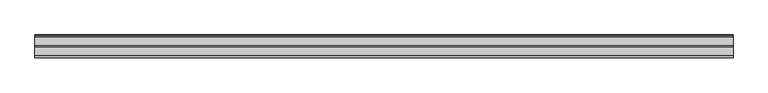
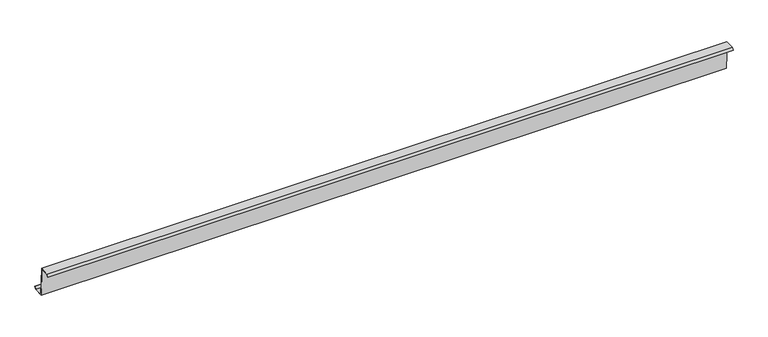
"""IFC4 building model written with IfcOpenShell, lengths in millimetres: proxy geometry, Generic Models 7:Generic Models 1:8:Generic Models 1:8 : Generic Models 7:Generic Models 1:337419:2 : Generic Models 7:Generic Models 1:8:Generic Models 1:8 : Generic Models 7:Generic Models 1:337419:315935."""

from ifc_helpers import new_model, si_unit, frame, origin, place, context, project, spatial, polyline, outline, extrude, source, transform, mapped, element, save


def generic_models_7addb1c7(model_context):
    return source(origin(), model_context, "Body", "SweptSolid", [
        extrude(outline(polyline([(-576223.748304, 4007.2948463), (-576158.9154956, 4009.9962133), (-576150.5718238, 3809.7480894), (-576089.8090698, 3812.2798708), (-576078.9727731, 3826.3439503), (-576076.7721093, 3824.6483508), (-576088.3990771, 3809.558085), (-576153.2318855, 3806.856718), (-576161.5755573, 4007.1048419), (-576222.3079951, 4004.5743236), (-576233.1561957, 3990.4947945), (-576235.3752717, 3992.2045805), (-576223.748304, 4007.2948463)])), frame((591306.0367239, 0.0, 0.0), z_axis=(1.0, 0.0, 0.0), x_axis=(0.0, 1.0, 0.0)), (0.0, 0.0, 1.0), 4876.8),
    ])


if __name__ == "__main__":
    model = new_model("IFC4")
    model_context = context("Model", 3, world=origin())
    ifc_project = project(units=[si_unit("LENGTHUNIT", "METRE", prefix="MILLI")], contexts=[model_context])
    site = spatial("IfcSite", under=ifc_project)
    building = spatial("IfcBuilding", under=site)
    placement = place(None, origin())
    generic_models_shape = generic_models_7addb1c7(model_context)
    element("IfcBuildingElementProxy", 1, Name="Generic Models 7:Generic Models 1:8:Generic Models 1:8 : Generic Models 7:Generic Models 1:337419:2 : Generic Models 7:Generic Models 1:8:Generic Models 1:8 : Generic Models 7:Generic Models 1:337419:315935", ObjectType="Generic Models 7:Generic Models 1:8:Generic Models 1:8 : Generic Models 7:Generic Models 1:337419:2 : Generic Models 7:Generic Models 1:8:Generic Models 1:8 : Generic Models 7:Generic Models 1:337419:315935", at=placement, inside=building, context=model_context, shape_type="MappedRepresentation", body=[
        mapped(generic_models_shape, transform((0.0, 0.0, 0.0), x_axis=(1.0, 0.0, 0.0), y_axis=(0.0, 1.0, 0.0), z_axis=(0.0, 0.0, 1.0))),
    ])
    save(model, "model.ifc")

# Revit data of these elements
# Type "Generic Models 7:Generic Models 1:8:Generic Models 1:8 : Generic Models 7:Generic Models 1:337419:2 : Generic Models 7:Generic Models 1:8:Generic Models 1:8 : Generic Models 7:Generic Models 1:337419:315935"
#   NameOverride = "Generic Models 7:Generic Models 1:8:Generic Models 1:8 : Generic Models 7:Generic Models 1:337419:315935"
#   ObjectTypeOverride = "Generic Models 1:8 : Generic Models 7:Generic Models 1:337419"
#   Reference = "Generic Models 1"
#   Tag = "315935"
# Element 1 (IfcBuildingElementProxy, "Generic Models 7:Generic Models 1:8:Generic Models 1:8 : Generic Models 7:Generic Models 1:337419:2 : Generic Models 7:Generic Models 1:8:Generic Models 1:8 : Generic Models 7:Generic Models 1:337419:315935")
#   Materials on its faces: "ZEE' PURLIN (SEE STRUCT. DWGS)"
# Materials
#   "ZEE' PURLIN (SEE STRUCT. DWGS)": class "Unassigned", colour RGB 210 209 208, transparency 0, Cost = 0
